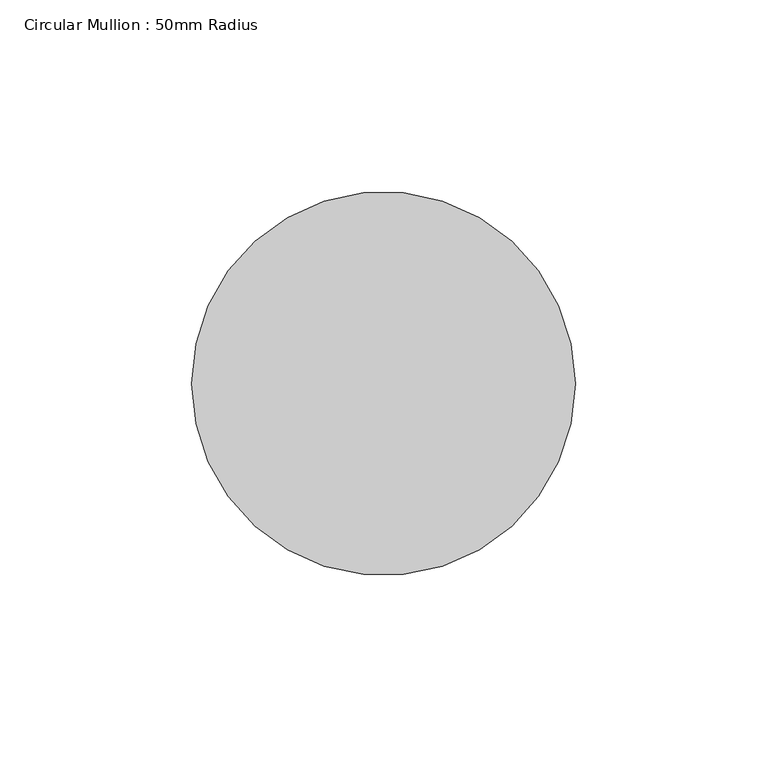
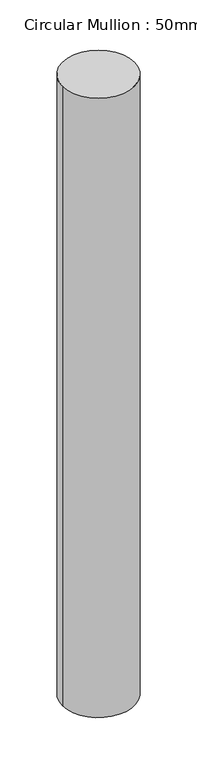
"""IFC4 building model written with IfcOpenShell, lengths in millimetres: member geometry, Circular Mullion : 50mm Radius."""

from ifc_helpers import new_model, si_unit, point, frame, origin, origin_2d, place, context, project, spatial, circle_curve, trimmed, segment, composite_curve, outline, extrude, source, transform, mapped, element, save


def circular_mullion_50mm_radius_9d536d19(model_context):
    return source(origin(), model_context, "Body", "SweptSolid", [
        extrude(outline(composite_curve([segment(trimmed(circle_curve(origin_2d(), 50.0), [point((50.0, 0.0))], [point((-50.0, 0.0))], False, "CARTESIAN"), True, "CONTINUOUS"), segment(trimmed(circle_curve(origin_2d(), 50.0), [point((-50.0, 0.0))], [point((50.0, 0.0))], False, "CARTESIAN"), True, "CONTINUOUS")], self_intersect=False)), frame((0.0, 0.0, -907.1221866), z_axis=(0.0, 0.0, 1.0), x_axis=(1.0, 0.0, 0.0)), (0.0, 0.0, 1.0), 907.1221866),
    ])


if __name__ == "__main__":
    model = new_model("IFC4")
    model_context = context("Model", 3, world=origin())
    ifc_project = project(units=[si_unit("LENGTHUNIT", "METRE", prefix="MILLI")], contexts=[model_context])
    site = spatial("IfcSite", under=ifc_project)
    building = spatial("IfcBuilding", under=site)
    placement = place(None, origin())
    circular_mullion_50mm_radius_shape = circular_mullion_50mm_radius_9d536d19(model_context)
    element("IfcMember", 1, ObjectType="Circular Mullion : 50mm Radius", at=placement, inside=building, context=model_context, shape_type="MappedRepresentation", body=[
        mapped(circular_mullion_50mm_radius_shape, transform((0.0, 0.0, 0.0), x_axis=(1.0, 0.0, 0.0), y_axis=(0.0, 1.0, 0.0), z_axis=(0.0, 0.0, 1.0))),
    ])
    save(model, "model.ifc")

# Revit data of these elements
# Type "Circular Mullion : 50mm Radius"
#   built-in parameter 1007350 = 0.164042 (stored number, unit not read)
# Element 1 (IfcMember, "Circular Mullion : 50mm Radius")
#   Materials on its faces: "Aluminium"
# Materials
#   "Aluminium": class "Metal", colour RGB 247 247 247, transparency 0, Description = "Aluminium 6061", Cost = 0
